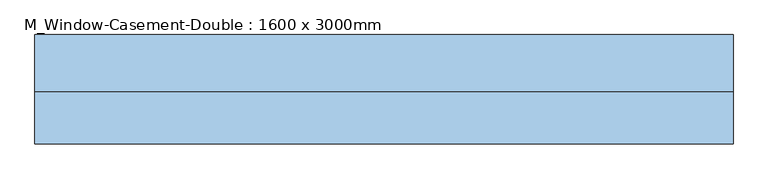
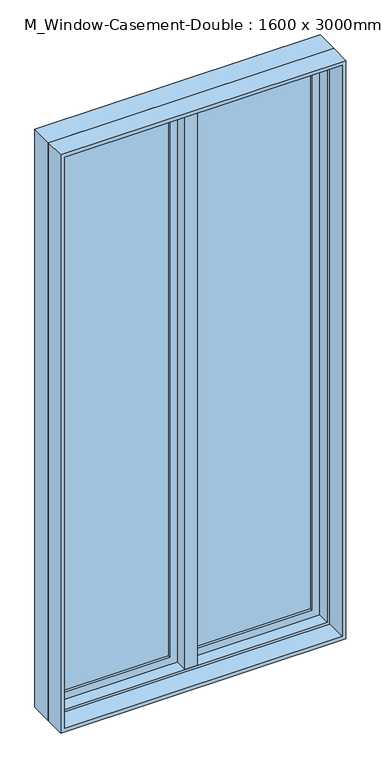
"""IFC4 building model written with IfcOpenShell, lengths in millimetres: window geometry, M_Window-Casement-Double : 1600 x 3000mm."""

from ifc_helpers import new_model, si_unit, frame, origin, place, context, project, spatial, polyline, outline, extrude, faceted_brep, source, transform, mapped, element, save


def m_window_casement_double_1600_x_3000mm_34ec59cd(model_context):
    return source(origin(), model_context, "Body", "SolidModel", [
        faceted_brep([(668.25, 68.25, 3868.25), (668.25, 4.75, 3868.25), (-668.25, 4.75, 3868.25), (-668.25, 68.25, 3868.25), (687.3, 119.05, 3887.3), (687.3, 68.25, 3887.3), (-687.3, 68.25, 3887.3), (-687.3, 119.05, 3887.3), (700.0, 4.75, 3900.0), (700.0, 119.05, 3900.0), (-700.0, 119.05, 3900.0), (-700.0, 4.75, 3900.0), (-668.25, 4.75, 931.75), (-668.25, 68.25, 931.75), (-687.3, 68.25, 912.7), (-687.3, 119.05, 912.7), (-700.0, 119.05, 900.0), (-700.0, 4.75, 900.0), (668.25, 4.75, 931.75), (668.25, 68.25, 931.75), (687.3, 68.25, 912.7), (687.3, 119.05, 912.7), (700.0, 119.05, 900.0), (700.0, 4.75, 900.0)], [[[0, 1, 2, 3]], [[4, 5, 6, 7]], [[8, 9, 10, 11]], [[3, 2, 12, 13]], [[7, 6, 14, 15]], [[11, 10, 16, 17]], [[13, 12, 18, 19]], [[15, 14, 20, 21]], [[17, 16, 22, 23]], [[11, 17, 23, 8], [1, 18, 12, 2]], [[19, 18, 1, 0]], [[5, 20, 14, 6], [3, 13, 19, 0]], [[21, 20, 5, 4]], [[23, 22, 9, 8]], [[9, 22, 16, 10], [7, 15, 21, 4]]]),
        extrude(outline(polyline([(3900.0, -700.0), (900.0, -700.0), (900.0, 700.0), (3900.0, 700.0), (3900.0, -700.0)]), holes=[polyline([(3880.95, 680.95), (919.05, 680.95), (919.05, -680.95), (3880.95, -680.95), (3880.95, 680.95)])]), frame((0.0, -100.0, 0.0), z_axis=(0.0, 1.0, 0.0), x_axis=(0.0, 0.0, 1.0)), (0.0, 0.0, 1.0), 104.75),
        extrude(outline(polyline([(912.7, 687.3), (3887.3, 687.3), (3887.3, 9.525), (912.7, 9.525), (912.7, 687.3)]), holes=[polyline([(969.85, 66.675), (3830.15, 66.675), (3830.15, 630.15), (969.85, 630.15), (969.85, 66.675)])]), frame((0.0, 68.25, 0.0), z_axis=(0.0, 1.0, 0.0), x_axis=(0.0, 0.0, 1.0)), (0.0, 0.0, 1.0), 44.45),
        extrude(outline(polyline([(3887.3, -687.3), (912.7, -687.3), (912.7, -9.525), (3887.3, -9.525), (3887.3, -687.3)]), holes=[polyline([(3830.15, -66.675), (969.85, -66.675), (969.85, -630.15), (3830.15, -630.15), (3830.15, -66.675)])]), frame((0.0, 68.25, 0.0), z_axis=(0.0, 1.0, 0.0), x_axis=(0.0, 0.0, 1.0)), (0.0, 0.0, 1.0), 44.45),
        extrude(outline(polyline([(630.15, 100.0), (630.15, 93.65), (66.675, 93.65), (66.675, 100.0), (630.15, 100.0)])), frame((0.0, 0.0, 969.85), z_axis=(0.0, 0.0, 1.0), x_axis=(1.0, 0.0, 0.0)), (0.0, 0.0, 1.0), 2860.3),
        extrude(outline(polyline([(66.675, 80.95), (66.675, 87.3), (630.15, 87.3), (630.15, 80.95), (66.675, 80.95)])), frame((0.0, 0.0, 969.85), z_axis=(0.0, 0.0, 1.0), x_axis=(1.0, 0.0, 0.0)), (0.0, 0.0, 1.0), 2860.3),
        extrude(outline(polyline([(-66.675, 100.0), (-66.675, 93.65), (-630.15, 93.65), (-630.15, 100.0), (-66.675, 100.0)])), frame((0.0, 0.0, 969.85), z_axis=(0.0, 0.0, 1.0), x_axis=(1.0, 0.0, 0.0)), (0.0, 0.0, 1.0), 2860.3),
        extrude(outline(polyline([(-630.15, 80.95), (-630.15, 87.3), (-66.675, 87.3), (-66.675, 80.95), (-630.15, 80.95)])), frame((0.0, 0.0, 969.85), z_axis=(0.0, 0.0, 1.0), x_axis=(1.0, 0.0, 0.0)), (0.0, 0.0, 1.0), 2860.3),
        faceted_brep([(9.525, 119.05, 3887.3), (-9.525, 119.05, 3887.3), (-9.525, 68.25, 3887.3), (9.525, 68.25, 3887.3), (9.525, 119.05, 912.7), (9.525, 68.25, 912.7), (-9.525, 68.25, 912.7), (-9.525, 119.05, 912.7), (-9.525, 68.25, 931.75), (-9.525, 68.25, 3868.25), (-30.1625, 68.25, 931.75), (-30.1625, 68.25, 3868.25), (-30.1625, 4.75, 931.75), (-30.1625, 4.75, 3868.25), (30.1625, 4.75, 931.75), (30.1625, 4.75, 3868.25), (30.1625, 68.25, 931.75), (30.1625, 68.25, 3868.25), (9.525, 68.25, 931.75), (9.525, 68.25, 3868.25)], [[[0, 1, 2, 3]], [[4, 5, 6, 7]], [[1, 0, 4, 7]], [[2, 1, 7, 6, 8, 9]], [[9, 8, 10, 11]], [[11, 10, 12, 13]], [[13, 12, 14, 15]], [[15, 14, 16, 17]], [[17, 16, 18, 19]], [[0, 3, 19, 18, 5, 4]], [[18, 8, 6, 5]], [[9, 19, 3, 2]], [[8, 18, 16, 14, 12, 10]], [[19, 9, 11, 13, 15, 17]]]),
    ])


if __name__ == "__main__":
    model = new_model("IFC4")
    model_context = context("Model", 3, world=origin())
    ifc_project = project(units=[si_unit("LENGTHUNIT", "METRE", prefix="MILLI")], contexts=[model_context])
    site = spatial("IfcSite", under=ifc_project)
    building = spatial("IfcBuilding", under=site)
    placement = place(None, origin())
    m_window_casement_double_1600_x_3000mm_shape = m_window_casement_double_1600_x_3000mm_34ec59cd(model_context)
    element("IfcWindow", 1, ObjectType="M_Window-Casement-Double : 1600 x 3000mm", at=placement, inside=building, context=model_context, shape_type="MappedRepresentation", body=[
        mapped(m_window_casement_double_1600_x_3000mm_shape, transform((0.0, 0.0, 0.0), x_axis=(1.0, 0.0, 0.0), y_axis=(0.0, 1.0, 0.0), z_axis=(0.0, 0.0, 1.0))),
    ])
    save(model, "model.ifc")

# Revit data of these elements
# Type "M_Window-Casement-Double : 1600 x 3000mm"
#   Type Mark = "39"
#   Fire Rating = "0.5h"
#   Analytic Construction = "Double glazing - domestic"
#   Frame Extension [instance default] = 6.35 mm
#   Window Inset [instance default] = 0 mm
#   Wall Thickness [instance default] = 150 mm
#   Interior Wall Closure [instance default] = 54.75 mm
#   Half Width = 700 mm
#   Visual Light Transmittance = 0.81
#   Thermal Resistance (R) = 0.319569 (m²·K)/W
#   Solar Heat Gain Coefficient = 0.76
#   Rough Width = 1415 mm
#   Rough Height = 3015 mm
#   Height = 3000 mm
#   Heat Transfer Coefficient (U) = 3.12929 W/(m²·K)
#   Exterior Wall Closure [instance default] = 31.8 mm
#   Extension Jamb [instance default] = 54.75 mm
#   Default Sill Height = 900 mm
#   Width = 1400 mm
#   Muntin Visibility = yes
#   Interior Trim Visibility [instance default] = yes
#   Exterior Trim Visibility [instance default] = yes
#   Extension Jamb Visibility [instance default] = yes
#   Interior Trim Material = Wood - Stained
#   Muntin Pattern = M_Muntin Pattern_2x2 : M_Muntin Pattern_2x2
#   Interior Trim = M_Trim-Window-Interior-Flat : Picture Frame
#   Interior Frame Material = Wood - Stained
#   Glass Panel Material = Glass
#   Exterior Trim Material = Clad - White
#   Exterior Trim = M_Trim-Window-Exterior-Flat : with Sill
#   Exterior Frame Material = Clad - White
#   Wall Closure = (empty or 0)
# Element 1 (IfcWindow, "M_Window-Casement-Double : 1600 x 3000mm")
#   Wall Thickness = 200 mm
#   Extension Jamb = 104.75 mm
#   Materials on its faces: "Wood - Stained", "Glass", "Clad - White"
# Materials
#   "Wood - Stained": class "Wood", colour RGB 173 132 96, transparency 0, Cost = 0
#   "Glass": class "Glass", colour RGB 245 245 243, transparency 1, Description = "Soda Lime Glass", Cost = 0
#   "Clad - White": class "Wood", colour RGB 245 245 243, transparency 0, Cost = 0
